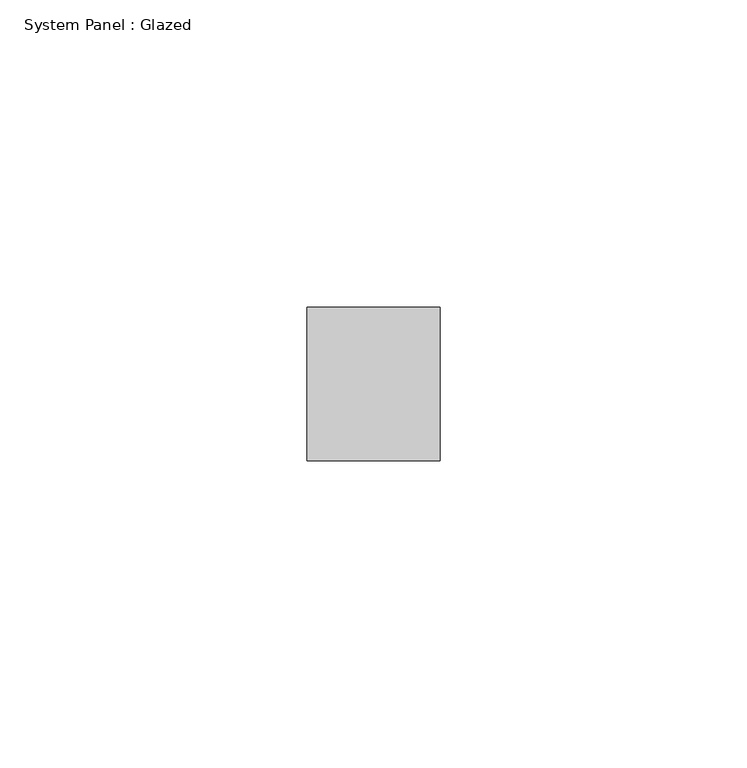
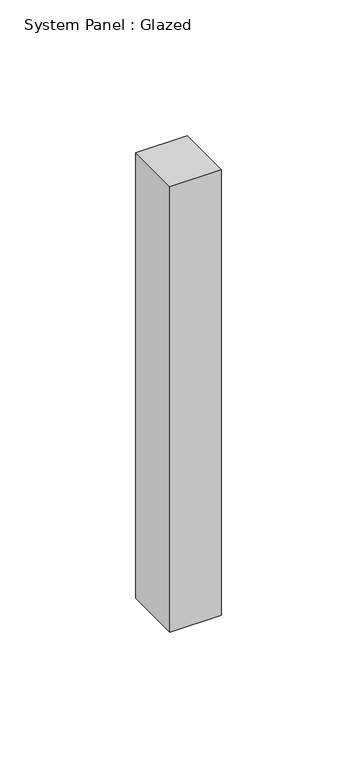
"""IFC4 building model written with IfcOpenShell, lengths in millimetres: plate geometry, System Panel : Glazed."""

from ifc_helpers import new_model, si_unit, origin, origin_with_axes, place, context, project, spatial, polyline, outline, extrude, source, transform, mapped, element, save


def system_panel_glazed_c2638314(model_context):
    return source(origin(), model_context, "Body", "SweptSolid", [
        extrude(outline(polyline([(10.8463273, 24.5), (-10.8463273, 24.5), (-10.8463273, 49.5), (10.8463273, 49.5), (10.8463273, 24.5)])), origin_with_axes(), (0.0, 0.0, 1.0), 200.0),
    ])


if __name__ == "__main__":
    model = new_model("IFC4")
    model_context = context("Model", 3, world=origin())
    ifc_project = project(units=[si_unit("LENGTHUNIT", "METRE", prefix="MILLI")], contexts=[model_context])
    site = spatial("IfcSite", under=ifc_project)
    building = spatial("IfcBuilding", under=site)
    placement = place(None, origin())
    system_panel_glazed_shape = system_panel_glazed_c2638314(model_context)
    element("IfcPlate", 1, ObjectType="System Panel : Glazed", at=placement, inside=building, context=model_context, shape_type="MappedRepresentation", body=[
        mapped(system_panel_glazed_shape, transform((0.0, 0.0, 0.0), x_axis=(1.0, 0.0, 0.0), y_axis=(0.0, 1.0, 0.0), z_axis=(0.0, 0.0, 1.0))),
    ])
    save(model, "model.ifc")

# Revit data of these elements
# Element 1 (IfcPlate, "System Panel : Glazed")
#   Materials on its faces: "Glass"
# Materials
#   "Glass": class "Glass", colour RGB 218 227 224, transparency 0.85, Description = "Soda Lime Glass", Cost = 0
